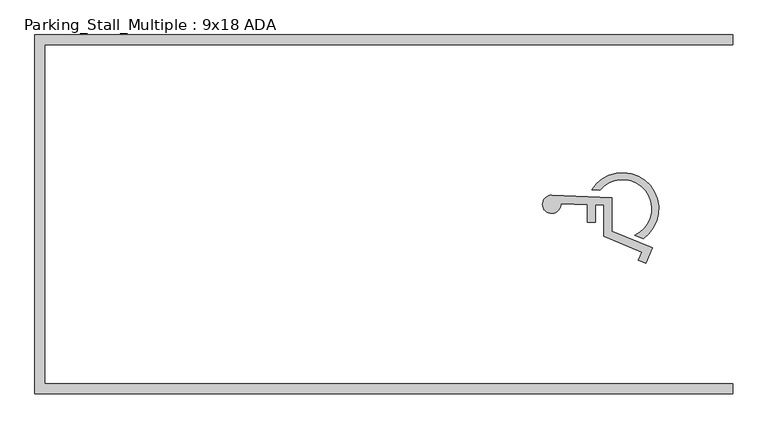
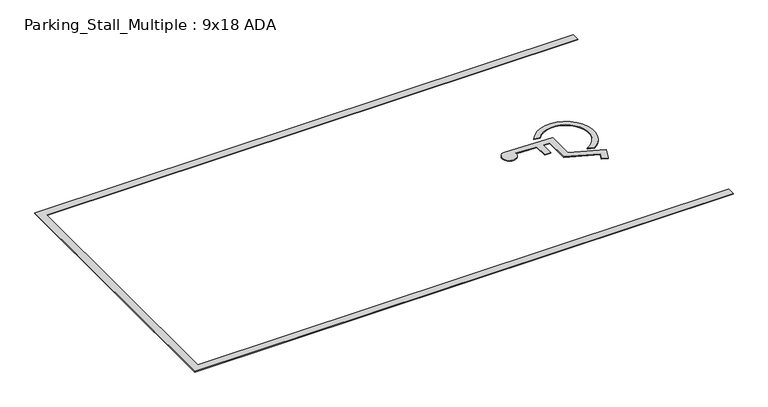
"""IFC4 building model written with IfcOpenShell, lengths in millimetres: proxy geometry, Parking_Stall_Multiple : 9x18 ADA."""

from ifc_helpers import new_model, si_unit, point, frame_2d, origin, origin_with_axes, place, context, project, spatial, polyline, circle_curve, trimmed, segment, composite_curve, outline, extrude, source, transform, mapped, element, save


def parking_stall_multiple_9x18_ada_f3c65445(model_context):
    return source(origin(), model_context, "Body", "SweptSolid", [
        extrude(outline(composite_curve([segment(trimmed(circle_curve(frame_2d((4063.0537792, 1487.7392135)), 71.682372), [point((4134.4870631, 1493.7098429))], [point((4065.8004874, 1559.3689423))], False, "CARTESIAN"), True, "CONTINUOUS"), segment(polyline([(4065.8004874, 1559.3689423), (4537.0669265, 1541.297795), (4537.0669265, 1277.7399509), (4855.5064238, 1147.2657706), (4804.6083075, 1023.3152993), (4746.1633873, 1047.3146946), (4773.0435548, 1112.7750627), (4473.8863941, 1235.3486933), (4473.8863941, 1480.5241666), (4407.514971, 1483.8792735), (4407.514971, 1348.7188556), (4344.3344387, 1348.7188556), (4344.3344387, 1486.3338395), (4134.4870631, 1493.7098429)]), True, "CONTINUOUS")], self_intersect=False)), origin_with_axes(), (0.0, 0.0, 1.0), 6.35),
        extrude(outline(composite_curve([segment(trimmed(circle_curve(frame_2d((4621.4451667, 1452.8961906)), 284.3262404), [point((4379.8123532, 1602.7460969))], [point((4782.6720114, 1218.7011532))], False, "CARTESIAN"), True, "CONTINUOUS"), segment(polyline([(4782.6720114, 1218.7011532), (4719.1799347, 1244.5051308)]), True, "CONTINUOUS"), segment(trimmed(circle_curve(frame_2d((4621.4451667, 1452.8961906)), 230.1714984), [point((4719.1799347, 1244.5051308))], [point((4443.3120901, 1598.661501))], True, "CARTESIAN"), True, "CONTINUOUS"), segment(polyline([(4443.3120901, 1598.661501), (4379.8123532, 1602.7460969)]), True, "CONTINUOUS")], self_intersect=False)), origin_with_axes(), (0.0, 0.0, 1.0), 6.35),
        extrude(outline(polyline([(5486.4, 0.0), (0.0, 0.0), (0.0, 2819.4), (5486.4, 2819.4), (5486.4, 2743.2), (76.2, 2743.2), (76.2, 76.2), (5486.4, 76.2), (5486.4, 0.0)])), origin_with_axes(), (0.0, 0.0, 1.0), 6.35),
    ])


if __name__ == "__main__":
    model = new_model("IFC4")
    model_context = context("Model", 3, world=origin())
    ifc_project = project(units=[si_unit("LENGTHUNIT", "METRE", prefix="MILLI")], contexts=[model_context])
    site = spatial("IfcSite", under=ifc_project)
    building = spatial("IfcBuilding", under=site)
    placement = place(None, origin())
    parking_stall_multiple_9x18_ada_shape = parking_stall_multiple_9x18_ada_f3c65445(model_context)
    element("IfcBuildingElementProxy", 1, Name="Parking_Stall_Multiple : 9x18 ADA", ObjectType="Parking_Stall_Multiple : 9x18 ADA", at=placement, inside=building, context=model_context, shape_type="MappedRepresentation", body=[
        mapped(parking_stall_multiple_9x18_ada_shape, transform((0.0, 0.0, 0.0), x_axis=(1.0, 0.0, 0.0), y_axis=(0.0, 1.0, 0.0), z_axis=(0.0, 0.0, 1.0))),
    ])
    save(model, "model.ifc")

# Revit data of these elements
# Type "Parking_Stall_Multiple : 9x18 ADA"
#   Parking_Width_M = 9' - 0"
#   Parking_Run_Length [instance default] = 65' - 0"
#   Parking_Line_Width = 0' - 3"
#   Parking_Length_M = 18' - 0"
#   Single_Parking_Visibility [instance default] = no
#   Parking_ADA_Symbol = yes
#   ParkingUnitsArray [instance default] = 7
#   ParkingUnits [instance default] = 7
#   Multiple_Parking_Visibility [instance default] = yes
#   Parking_Line_Material = none
# Element 1 (IfcBuildingElementProxy, "Parking_Stall_Multiple : 9x18 ADA")
#   Parking_Run_Length = 8' - 10 1/2"
#   Single_Parking_Visibility = yes
#   ParkingUnitsArray = 2
#   ParkingUnits = 1
#   Multiple_Parking_Visibility = no
